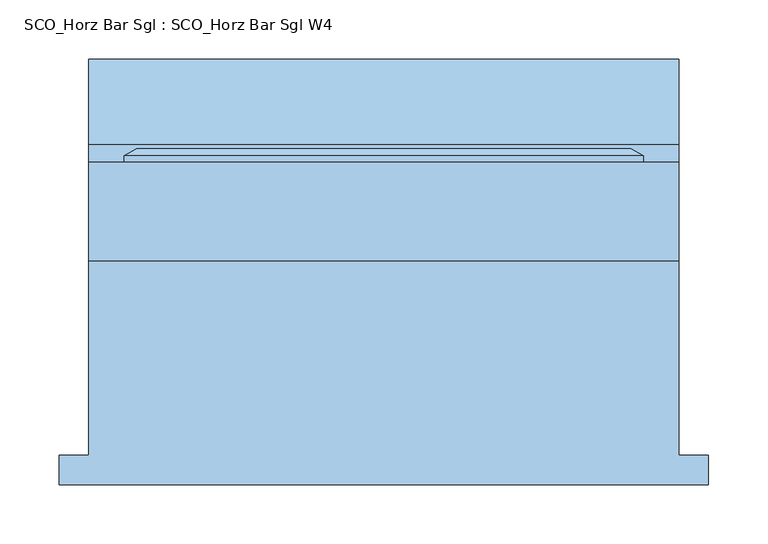
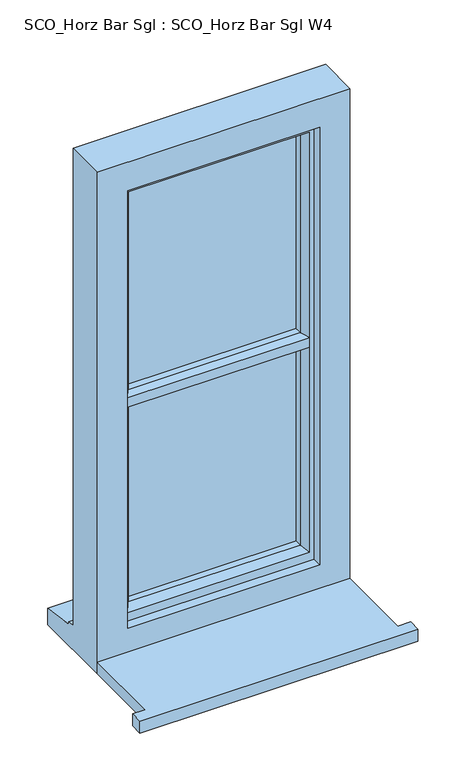
"""IFC4 building model written with IfcOpenShell, lengths in millimetres: window geometry, SCO_Horz Bar Sgl : SCO_Horz Bar Sgl W4."""

from ifc_helpers import new_model, si_unit, frame, origin, place, context, project, spatial, polyline, outline, extrude, faceted_brep, source, transform, mapped, element, save


def sco_horz_bar_sgl_sco_horz_bar_sgl_w4_ff072667(model_context):
    return source(origin(), model_context, "Body", "SolidModel", [
        extrude(outline(polyline([(-275.0, -191.5434322), (-275.0, -166.5434322), (-250.0, -166.5434322), (-250.0, -2.0434322), (250.0, -2.0434322), (250.0, -166.5434322), (275.0, -166.5434322), (275.0, -191.5434322), (-275.0, -191.5434322)])), frame((0.0, 0.0, 1060.0), z_axis=(0.0, 0.0, 1.0), x_axis=(1.0, 0.0, 0.0)), (0.0, 0.0, 1.0), 25.0),
        faceted_brep([(-250.0, -2.0434322, 1060.0), (250.0, -2.0434322, 1060.0), (250.0, -2.0434322, 2110.0), (-250.0, -2.0434322, 2110.0), (-190.0, -2.0434322, 2050.0), (190.0, -2.0434322, 2050.0), (190.0, -2.0434322, 1135.0), (-190.0, -2.0434322, 1135.0), (-250.0, 80.9565678, 2110.0), (-250.0, 80.9565678, 1111.0), (-250.0, 95.9565678, 1109.68767), (-250.0, 95.9565678, 1104.7449676), (-250.0, 168.4565678, 1093.8088847), (-250.0, 168.4565678, 1060.0), (250.0, 80.9565678, 2110.0), (250.0, 80.9565678, 1111.0), (-210.0, 80.9565678, 2070.0), (-210.0, 80.9565678, 1123.0), (210.0, 80.9565678, 1123.0), (210.0, 80.9565678, 2070.0), (-210.0, 15.9565678, 2070.0), (-210.0, 15.9565678, 1123.0), (210.0, 15.9565678, 2070.0), (210.0, 15.9565678, 1123.0), (-190.0, 15.9565678, 2050.0), (-190.0, 15.9565678, 1135.0), (190.0, 15.9565678, 1135.0), (190.0, 15.9565678, 2050.0), (250.0, 168.4565678, 1060.0), (250.0, 168.4565678, 1093.8088847), (250.0, 95.9565678, 1104.7449676), (250.0, 95.9565678, 1109.68767)], [[[0, 1, 2, 3], [4, 5, 6, 7]], [[0, 3, 8, 9, 10, 11, 12, 13]], [[9, 8, 14, 15], [16, 17, 18, 19]], [[17, 16, 20, 21]], [[20, 22, 23, 21], [24, 25, 26, 27]], [[24, 4, 7, 25]], [[3, 2, 14, 8]], [[16, 19, 22, 20]], [[5, 4, 24, 27]], [[15, 14, 2, 1, 28, 29, 30, 31]], [[19, 18, 23, 22]], [[5, 27, 26, 6]], [[28, 1, 0, 13]], [[29, 28, 13, 12]], [[30, 29, 12, 11]], [[31, 30, 11, 10]], [[15, 31, 10, 9]], [[21, 23, 18, 17]], [[7, 6, 26, 25]]]),
        extrude(outline(polyline([(180.1480377, 44.9565678), (-180.0, 44.9565678), (-180.0, 68.9565678), (180.1480377, 68.9565678), (180.1480377, 44.9565678)])), frame((0.0, 0.0, 1153.0), z_axis=(0.0, 0.0, 1.0), x_axis=(1.0, 0.0, 0.0)), (0.0, 0.0, 1.0), 434.3307627),
        extrude(outline(polyline([(180.1480377, 44.9565678), (-180.0, 44.9565678), (-180.0, 68.9565678), (180.1480377, 68.9565678), (180.1480377, 44.9565678)])), frame((0.0, 0.0, 1597.6692373), z_axis=(0.0, 0.0, 1.0), x_axis=(1.0, 0.0, 0.0)), (0.0, 0.0, 1.0), 442.3307627),
        extrude(outline(polyline([(92.5035732, 1597.6692373), (92.5035732, 1587.3307627), (86.8277797, 1577.5), (68.9565678, 1577.5), (68.9565678, 1584.5), (44.9565678, 1584.5), (44.9565678, 1577.5), (30.4494677, 1577.5), (15.9565678, 1582.6480377), (15.9565678, 1602.3519623), (30.4494677, 1607.5), (44.9565678, 1607.5), (44.9565678, 1600.5), (68.9565678, 1600.5), (68.9565678, 1607.5), (86.8277797, 1607.5), (92.5035732, 1597.6692373)])), frame((-180.1480377, 0.0, 0.0), z_axis=(1.0, 0.0, 0.0), x_axis=(0.0, 1.0, 0.0)), (0.0, 0.0, 1.0), 360.2960754),
        faceted_brep([(-220.0, 80.9565678, 2072.0), (-220.0, 86.7300705, 2072.0), (-220.0, 86.7300705, 1113.0), (-220.0, 80.9565678, 1113.0), (-210.0, 15.9565678, 2062.0), (-210.0, 80.9565678, 2062.0), (-210.0, 80.9565678, 1123.0), (-210.0, 15.9565678, 1123.0), (-170.0, 30.4494677, 2022.0), (-180.1480377, 15.9565678, 2032.1480377), (-180.1480377, 15.9565678, 1152.8519623), (-170.0, 30.4494677, 1163.0), (-170.0, 44.9565678, 2022.0), (-170.0, 44.9565678, 1163.0), (-180.0, 68.9565678, 2032.0), (-180.0, 44.9565678, 2032.0), (-180.0, 44.9565678, 1153.0), (-180.0, 68.9565678, 1153.0), (-170.0, 86.7300705, 2022.0), (-170.0, 68.9565678, 2022.0), (-170.0, 68.9565678, 1163.0), (-170.0, 86.7300705, 1163.0), (-180.0, 92.5035732, 2032.0), (-180.0, 92.5035732, 1153.0), (-209.2153903, 92.5035732, 2061.2153903), (-209.2153903, 92.5035732, 1123.7846097), (220.0, 86.7300705, 1113.0), (220.0, 80.9565678, 1113.0), (210.0, 80.9565678, 1123.0), (210.0, 15.9565678, 1123.0), (180.1480377, 15.9565678, 1152.8519623), (170.0, 30.4494677, 1163.0), (170.0, 44.9565678, 1163.0), (180.0, 44.9565678, 1153.0), (180.0, 68.9565678, 1153.0), (170.0, 68.9565678, 1163.0), (170.0, 86.7300705, 1163.0), (180.0, 92.5035732, 1153.0), (209.2153903, 92.5035732, 1123.7846097), (220.0, 86.7300705, 2072.0), (220.0, 80.9565678, 2072.0), (210.0, 80.9565678, 2062.0), (210.0, 15.9565678, 2062.0), (180.1480377, 15.9565678, 2032.1480377), (170.0, 30.4494677, 2022.0), (170.0, 44.9565678, 2022.0), (180.0, 44.9565678, 2032.0), (180.0, 68.9565678, 2032.0), (170.0, 68.9565678, 2022.0), (170.0, 86.7300705, 2022.0), (180.0, 92.5035732, 2032.0), (209.2153903, 92.5035732, 2061.2153903)], [[[0, 1, 2, 3]], [[4, 5, 6, 7]], [[8, 9, 10, 11]], [[12, 8, 11, 13]], [[14, 15, 16, 17]], [[18, 19, 20, 21]], [[22, 18, 21, 23]], [[1, 24, 25, 2]], [[3, 2, 26, 27]], [[7, 6, 28, 29]], [[11, 10, 30, 31]], [[13, 11, 31, 32]], [[17, 16, 33, 34]], [[21, 20, 35, 36]], [[23, 21, 36, 37]], [[2, 25, 38, 26]], [[27, 26, 39, 40]], [[29, 28, 41, 42]], [[31, 30, 43, 44]], [[32, 31, 44, 45]], [[34, 33, 46, 47]], [[36, 35, 48, 49]], [[37, 36, 49, 50]], [[26, 38, 51, 39]], [[40, 39, 1, 0]], [[3, 27, 40, 0], [5, 41, 28, 6]], [[42, 41, 5, 4]], [[7, 29, 42, 4], [9, 43, 30, 10]], [[44, 43, 9, 8]], [[45, 44, 8, 12]], [[15, 46, 33, 16], [13, 32, 45, 12]], [[47, 46, 15, 14]], [[17, 34, 47, 14], [19, 48, 35, 20]], [[49, 48, 19, 18]], [[50, 49, 18, 22]], [[24, 51, 38, 25], [23, 37, 50, 22]], [[39, 51, 24, 1]]]),
    ])


if __name__ == "__main__":
    model = new_model("IFC4")
    model_context = context("Model", 3, world=origin())
    ifc_project = project(units=[si_unit("LENGTHUNIT", "METRE", prefix="MILLI")], contexts=[model_context])
    site = spatial("IfcSite", under=ifc_project)
    building = spatial("IfcBuilding", under=site)
    placement = place(None, origin())
    sco_horz_bar_sgl_sco_horz_bar_sgl_w4_shape = sco_horz_bar_sgl_sco_horz_bar_sgl_w4_ff072667(model_context)
    element("IfcWindow", 1, ObjectType="SCO_Horz Bar Sgl : SCO_Horz Bar Sgl W4", at=placement, inside=building, context=model_context, shape_type="MappedRepresentation", body=[
        mapped(sco_horz_bar_sgl_sco_horz_bar_sgl_w4_shape, transform((0.0, 0.0, 0.0), x_axis=(1.0, 0.0, 0.0), y_axis=(0.0, 1.0, 0.0), z_axis=(0.0, 0.0, 1.0))),
    ])
    save(model, "model.ifc")

# Revit data of these elements
# Type "SCO_Horz Bar Sgl : SCO_Horz Bar Sgl W4"
#   Type Mark = "W4"
#   Operation = "SinglePanel"
#   Manufacturer = "Revit"
#   Keynote = "L10"
#   Wrap Layers (Ext) from Ext = 102.5 mm
#   Wrap Layers (Int) from Ext = 177.5 mm
#   Window Board Projection = 25 mm
#   Window Board Extension = 25 mm
#   Rough Width = 500 mm
#   Rough Height = 1050 mm
#   Height = 1050 mm
#   Width = 500 mm
#   Glazing Thickness = 24 mm
#   FrameOffset - External = 102.5 mm
#   Frame Depth = 65 mm
#   Ext Leaf Thickness (Scot) = 102.5 mm
#   Ext Leaf Overlap (Scot) = 25 mm
#   Default Head Height = 2110 mm
#   Cill Depth = 87.5 mm
#   Cavity Closer Width = 50 mm
#   Cavity Closer Offset from Ext = 102.5 mm
#   Cavity Closer Depth = 85 mm
#   Vis - Cavity Closers = yes
#   Material Trim = Window Frame
#   Material Glass = Glass
#   Material Frame = Window Frame
#   Wall Closure = (empty or 0)
# Element 1 (IfcWindow, "SCO_Horz Bar Sgl : SCO_Horz Bar Sgl W4")
#   Materials on its faces: "Window Frame", "Glass"
# Materials
#   "Window Frame": class "Miscellaneous", colour RGB 249 249 249, transparency 0
#   "Glass": class "Glass", colour RGB 0 128 192, transparency 0.75
